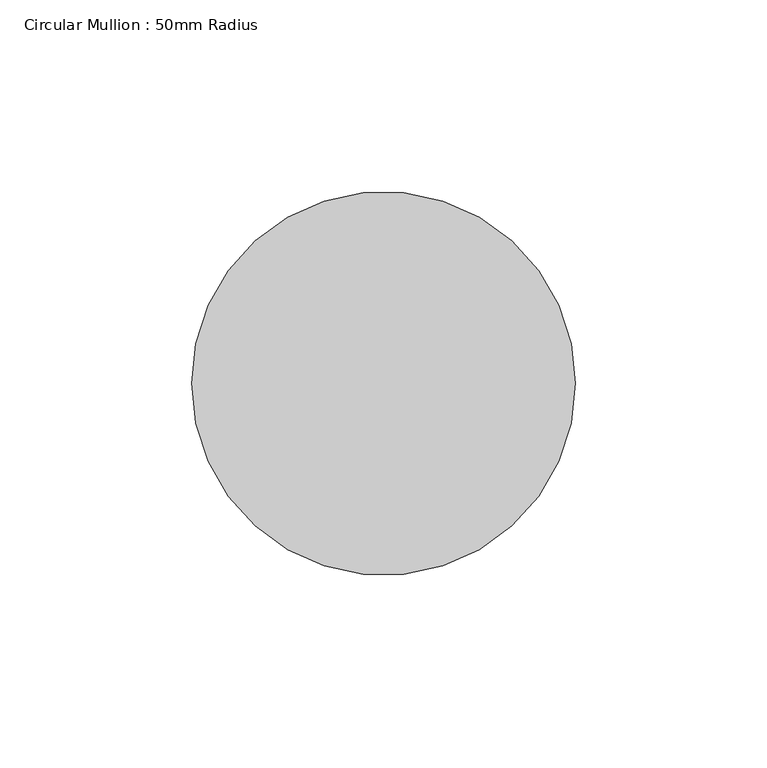
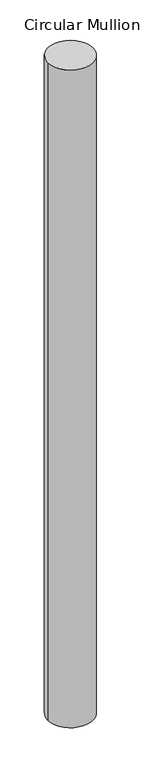
"""IFC4 building model written with IfcOpenShell, lengths in millimetres: member geometry, Circular Mullion : 50mm Radius."""

from ifc_helpers import new_model, si_unit, point, frame, origin, origin_2d, place, context, project, spatial, circle_curve, trimmed, segment, composite_curve, outline, extrude, source, transform, mapped, element, save


def circular_mullion_50mm_radius_4a66e798(model_context):
    return source(origin(), model_context, "Body", "SweptSolid", [
        extrude(outline(composite_curve([segment(trimmed(circle_curve(origin_2d(), 50.0), [point((50.0, 0.0))], [point((-50.0, 0.0))], False, "CARTESIAN"), True, "CONTINUOUS"), segment(trimmed(circle_curve(origin_2d(), 50.0), [point((-50.0, 0.0))], [point((50.0, 0.0))], False, "CARTESIAN"), True, "CONTINUOUS")], self_intersect=False)), frame((0.0, 0.0, -1544.0275175), z_axis=(0.0, 0.0, 1.0), x_axis=(1.0, 0.0, 0.0)), (0.0, 0.0, 1.0), 1544.0275175),
    ])


if __name__ == "__main__":
    model = new_model("IFC4")
    model_context = context("Model", 3, world=origin())
    ifc_project = project(units=[si_unit("LENGTHUNIT", "METRE", prefix="MILLI")], contexts=[model_context])
    site = spatial("IfcSite", under=ifc_project)
    building = spatial("IfcBuilding", under=site)
    placement = place(None, origin())
    circular_mullion_50mm_radius_shape = circular_mullion_50mm_radius_4a66e798(model_context)
    element("IfcMember", 1, ObjectType="Circular Mullion : 50mm Radius", at=placement, inside=building, context=model_context, shape_type="MappedRepresentation", body=[
        mapped(circular_mullion_50mm_radius_shape, transform((0.0, 0.0, 0.0), x_axis=(1.0, 0.0, 0.0), y_axis=(0.0, 1.0, 0.0), z_axis=(0.0, 0.0, 1.0))),
    ])
    save(model, "model.ifc")

# Revit data of these elements
# Type "Circular Mullion : 50mm Radius"
#   built-in parameter 1007350 = 0.164042 (stored number, unit not read)
# Element 1 (IfcMember, "Circular Mullion : 50mm Radius")
#   Materials on its faces: "Aluminium"
# Materials
#   "Aluminium": class "Metal", colour RGB 247 247 247, transparency 0, Description = "Aluminium 6061", Cost = 0
